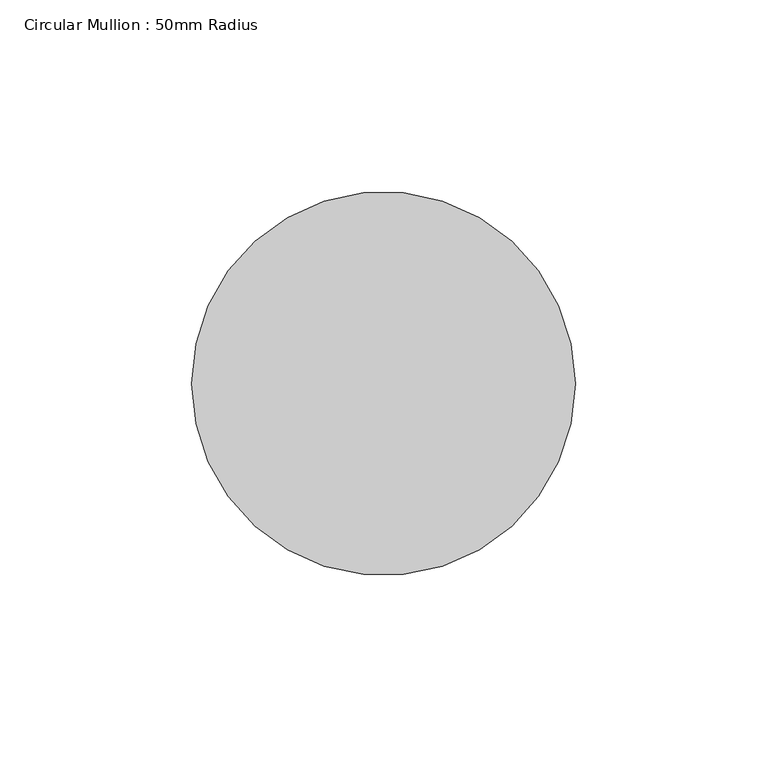
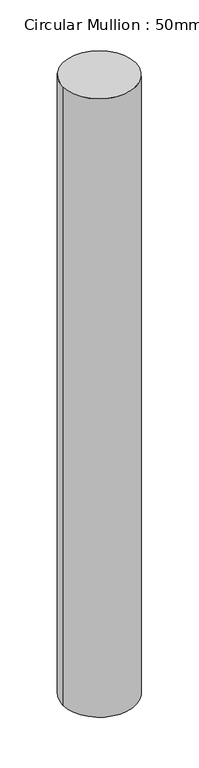
"""IFC4 building model written with IfcOpenShell, lengths in millimetres: member geometry, Circular Mullion : 50mm Radius."""

import ifcopenshell
import ifcopenshell.guid

model = None  # the IFC model being written
_history = None  # IfcOwnerHistory: only IFC2X3 demands one
_inside = {}  # id of a spatial element -> (the spatial element, [elements in it])
_under = {}  # id of a project, library or spatial element -> (it, [spatial elements below it])
_declared = {}  # id of a project -> (the project, [libraries it declares])
_typed = {}  # id of a type object -> (the type object, [elements of that type])
_made_of = {}  # id of a material, layer set ... -> (it, [elements and type objects made of it])


def new_model(schema):
    """Start an empty IFC model of exactly this schema.

    Asked for "IFC4X3", IfcOpenShell would pick the latest addendum, in which some entities
    have other attributes; the version numbers below select the first issue.
    IFC2X3 requires an IfcOwnerHistory on every rooted entity: one is made here for all.
    """
    global model, _history
    if schema == "IFC4X3":
        model = ifcopenshell.file(schema_version=(4, 3, 0, 0))
    else:
        model = ifcopenshell.file(schema=schema)
    _inside.clear()
    _under.clear()
    _declared.clear()
    _typed.clear()
    _made_of.clear()
    _history = None
    if model.schema == "IFC2X3":
        org = make("IfcOrganization", Name="unknown")
        user = make(
            "IfcPersonAndOrganization",
            ThePerson=make("IfcPerson", FamilyName="unknown"),
            TheOrganization=org,
        )
        app = make(
            "IfcApplication",
            ApplicationDeveloper=org,
            Version="unknown",
            ApplicationFullName="unknown",
            ApplicationIdentifier="unknown",
        )
        _history = make(
            "IfcOwnerHistory",
            OwningUser=user,
            OwningApplication=app,
            ChangeAction="ADDED",
            CreationDate=0,
        )
    return model


def make(cls, **values):
    """One entity of the class cls with the attributes given. An attribute that is None is left unset."""
    return model.create_entity(
        cls, **{name: value for name, value in values.items() if value is not None}
    )


def rooted(cls, **values):
    """An entity with a GlobalId (a new one), such as an element, a storey or a relation."""
    return make(cls, GlobalId=ifcopenshell.guid.new(), OwnerHistory=_history, **values)


def si_unit(unit_type, name, prefix=None):
    """IfcSIUnit, for example si_unit("LENGTHUNIT", "METRE", prefix="MILLI")."""
    return make("IfcSIUnit", UnitType=unit_type, Prefix=prefix, Name=name)


def assignment(units):
    """IfcUnitAssignment: the units of a project."""
    return None if units is None else make("IfcUnitAssignment", Units=units)


def point(xyz):
    """IfcCartesianPoint."""
    return None if xyz is None else make("IfcCartesianPoint", Coordinates=xyz)


def direction(xyz):
    """IfcDirection."""
    return None if xyz is None else make("IfcDirection", DirectionRatios=xyz)


def frame(location, z_axis=None, x_axis=None):
    """IfcAxis2Placement3D, a coordinate frame: its origin and axes. An axis left out is left unset."""
    return make(
        "IfcAxis2Placement3D",
        Location=point(location),
        Axis=direction(z_axis),
        RefDirection=direction(x_axis),
    )


def frame_2d(location, x_axis=None):
    """IfcAxis2Placement2D, a coordinate frame in the plane: its origin and x axis."""
    return make(
        "IfcAxis2Placement2D", Location=point(location), RefDirection=direction(x_axis)
    )


def origin():
    """The frame at (0, 0, 0) with its axes left unset."""
    return frame((0.0, 0.0, 0.0))


def origin_2d():
    """The frame at (0, 0) in the plane with its x axis left unset."""
    return frame_2d((0.0, 0.0))


def place(relative_to, where):
    """IfcLocalPlacement: puts the frame where relative to a parent placement (None: the world)."""
    return make(
        "IfcLocalPlacement", PlacementRelTo=relative_to, RelativePlacement=where
    )


def context(
    kind, dimensions, precision=None, world=None, true_north=None, identifier=None
):
    """IfcGeometricRepresentationContext, for example the 3D "Model" context."""
    return make(
        "IfcGeometricRepresentationContext",
        ContextIdentifier=identifier,
        ContextType=kind,
        CoordinateSpaceDimension=dimensions,
        Precision=precision,
        WorldCoordinateSystem=world,
        TrueNorth=true_north,
    )


def project(units=None, contexts=None):
    """IfcProject with its units and contexts."""
    return rooted(
        "IfcProject",
        Name="project",
        RepresentationContexts=contexts,
        UnitsInContext=assignment(units),
    )


def spatial(cls, under=None, at=None, **own):
    """A site, building, storey or space (cls), placed at a placement, below another one or the project."""
    s = rooted(cls, ObjectPlacement=at, **own)
    if under is not None:
        _under.setdefault(under.id(), (under, []))[1].append(s)
    return s


def circle_curve(where, radius):
    """IfcCircle in the frame where."""
    return make("IfcCircle", Position=where, Radius=radius)


def trimmed(basis, trim1, trim2, sense, master):
    """IfcTrimmedCurve: the piece of a basis curve between two trims."""
    return make(
        "IfcTrimmedCurve",
        BasisCurve=basis,
        Trim1=trim1,
        Trim2=trim2,
        SenseAgreement=sense,
        MasterRepresentation=master,
    )


def segment(curve, same_sense, transition):
    """IfcCompositeCurveSegment."""
    return make(
        "IfcCompositeCurveSegment",
        Transition=transition,
        SameSense=same_sense,
        ParentCurve=curve,
    )


def composite_curve(segments, self_intersect=None):
    """IfcCompositeCurve: segments joined end to end."""
    return make("IfcCompositeCurve", Segments=segments, SelfIntersect=self_intersect)


def outline(outer, holes=None, kind="AREA"):
    """IfcArbitraryClosedProfileDef: a profile drawn as a closed curve; with holes, ...WithVoids."""
    if holes is None:
        return make("IfcArbitraryClosedProfileDef", ProfileType=kind, OuterCurve=outer)
    return make(
        "IfcArbitraryProfileDefWithVoids",
        ProfileType=kind,
        OuterCurve=outer,
        InnerCurves=holes,
    )


def extrude(swept, where, along, depth):
    """IfcExtrudedAreaSolid: the profile swept, set in the frame where, extruded along a direction by depth."""
    return make(
        "IfcExtrudedAreaSolid",
        SweptArea=swept,
        Position=where,
        ExtrudedDirection=direction(along),
        Depth=depth,
    )


def shape(context_of_items, identifier, shape_type, items):
    """IfcShapeRepresentation: the items that make up one representation, for example the "Body"."""
    return make(
        "IfcShapeRepresentation",
        ContextOfItems=context_of_items,
        RepresentationIdentifier=identifier,
        RepresentationType=shape_type,
        Items=items,
    )


def source(mapping_origin, context_of_items, identifier, shape_type, items):
    """IfcRepresentationMap: a shape defined once, which mapped items show again and again."""
    return make(
        "IfcRepresentationMap",
        MappingOrigin=mapping_origin,
        MappedRepresentation=shape(context_of_items, identifier, shape_type, items),
    )


def transform(
    local_origin,
    x_axis=None,
    y_axis=None,
    z_axis=None,
    scale=None,
    scale2=None,
    scale3=None,
    uniform=True,
):
    """IfcCartesianTransformationOperator3D, or its non-uniform kind. x_axis, y_axis, z_axis: its Axis1, 2, 3."""
    if uniform:
        return make(
            "IfcCartesianTransformationOperator3D",
            Axis1=direction(x_axis),
            Axis2=direction(y_axis),
            LocalOrigin=point(local_origin),
            Scale=scale,
            Axis3=direction(z_axis),
        )
    return make(
        "IfcCartesianTransformationOperator3DnonUniform",
        Axis1=direction(x_axis),
        Axis2=direction(y_axis),
        LocalOrigin=point(local_origin),
        Scale=scale,
        Axis3=direction(z_axis),
        Scale2=scale2,
        Scale3=scale3,
    )


def mapped(mapping_source, mapping_target):
    """IfcMappedItem: shows the shape of a source again, moved by a transform."""
    return make(
        "IfcMappedItem", MappingSource=mapping_source, MappingTarget=mapping_target
    )


def made_of(thing, what):
    """Note that an element or type object is made of a material, layer set ...; save() writes the relation."""
    if what is not None:
        _made_of.setdefault(what.id(), (what, []))[1].append(thing)
    return thing


def element(
    cls,
    number,
    at=None,
    inside=None,
    cuts=None,
    type_object=None,
    material=None,
    context=None,
    identifier="Body",
    shape_type=None,
    held_by="IfcProductDefinitionShape",
    body=None,
    shapes=None,
    **own,
):
    """One element of the class cls, such as IfcWall. Its Tag is "e" and its number.

    at: its placement. inside: the storey or other place that contains it. cuts: it is an
    opening in that element (IfcRelVoidsElement). A single representation is given by context,
    identifier, shape_type and body (its items); several are given by shapes. held_by: the class
    of the entity that holds the representations. save() writes the other relations.
    """
    e = rooted(cls, Tag="e%d" % number, ObjectPlacement=at, **own)
    if body is not None:
        shapes = [shape(context, identifier, shape_type, body)]
    if shapes is not None:
        e.Representation = make(held_by, Representations=shapes)
    if inside is not None:
        _inside.setdefault(inside.id(), (inside, []))[1].append(e)
    if cuts is not None:
        rooted(
            "IfcRelVoidsElement", RelatingBuildingElement=cuts, RelatedOpeningElement=e
        )
    if type_object is not None:
        _typed.setdefault(type_object.id(), (type_object, []))[1].append(e)
    return made_of(e, material)


def aggregate(whole, parts):
    """IfcRelAggregates: a whole, such as a stair, and the parts it consists of."""
    return rooted("IfcRelAggregates", RelatingObject=whole, RelatedObjects=parts)


def save(model, path):
    """Write the relations noted so far, then the file.

    IfcRelAggregates (storeys below a building ...), IfcRelContainedInSpatialStructure (elements
    in a storey), IfcRelDefinesByType, IfcRelAssociatesMaterial and IfcRelDeclares: one each for
    every whole, place, type object, material and project.
    """
    for whole, parts in _under.values():
        aggregate(whole, parts)
    for where, things in _inside.values():
        rooted(
            "IfcRelContainedInSpatialStructure",
            RelatedElements=things,
            RelatingStructure=where,
        )
    for kind, things in _typed.values():
        rooted("IfcRelDefinesByType", RelatedObjects=things, RelatingType=kind)
    for what, things in _made_of.values():
        rooted("IfcRelAssociatesMaterial", RelatedObjects=things, RelatingMaterial=what)
    for by, libraries in _declared.values():
        rooted("IfcRelDeclares", RelatingContext=by, RelatedDefinitions=libraries)
    model.write(path)


def circular_mullion_50mm_radius_12fe219f(model_context):
    return source(origin(), model_context, "Body", "SweptSolid", [
        extrude(outline(composite_curve([segment(trimmed(circle_curve(origin_2d(), 50.0), [point((50.0, 0.0))], [point((-50.0, 0.0))], False, "CARTESIAN"), True, "CONTINUOUS"), segment(trimmed(circle_curve(origin_2d(), 50.0), [point((-50.0, 0.0))], [point((50.0, 0.0))], False, "CARTESIAN"), True, "CONTINUOUS")], self_intersect=False)), frame((0.0, 0.0, -899.6731502), z_axis=(0.0, 0.0, 1.0), x_axis=(1.0, 0.0, 0.0)), (0.0, 0.0, 1.0), 899.6731502),
    ])


if __name__ == "__main__":
    model = new_model("IFC4")
    model_context = context("Model", 3, world=origin())
    ifc_project = project(units=[si_unit("LENGTHUNIT", "METRE", prefix="MILLI")], contexts=[model_context])
    site = spatial("IfcSite", under=ifc_project)
    building = spatial("IfcBuilding", under=site)
    placement = place(None, origin())
    circular_mullion_50mm_radius_shape = circular_mullion_50mm_radius_12fe219f(model_context)
    element("IfcMember", 1, ObjectType="Circular Mullion : 50mm Radius", at=placement, inside=building, context=model_context, shape_type="MappedRepresentation", body=[
        mapped(circular_mullion_50mm_radius_shape, transform((0.0, 0.0, 0.0), x_axis=(1.0, 0.0, 0.0), y_axis=(0.0, 1.0, 0.0), z_axis=(0.0, 0.0, 1.0))),
    ])
    save(model, "model.ifc")

# Revit data of these elements
# Type "Circular Mullion : 50mm Radius"
#   built-in parameter 1007350 = 0.164042 (stored number, unit not read)
# Element 1 (IfcMember, "Circular Mullion : 50mm Radius")
#   Materials on its faces: "Aluminium"
# Materials
#   "Aluminium": class "Metal", colour RGB 247 247 247, transparency 0, Description = "Aluminium 6061", Cost = 0
